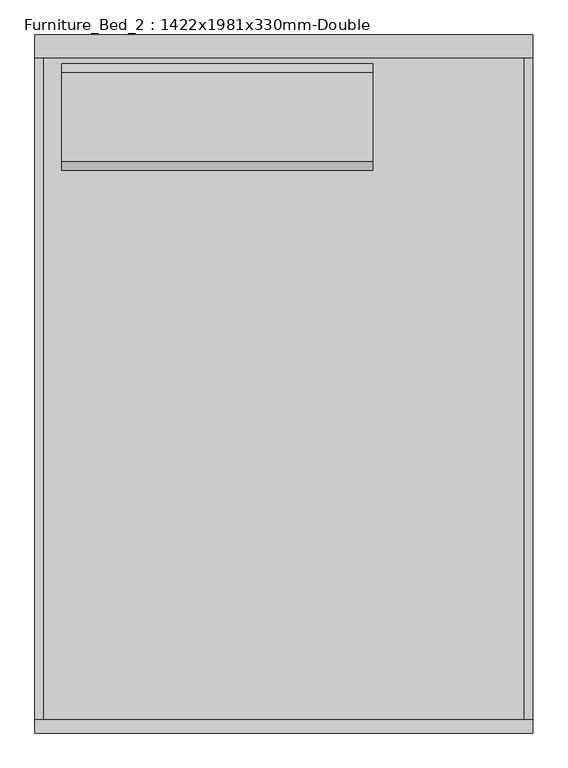
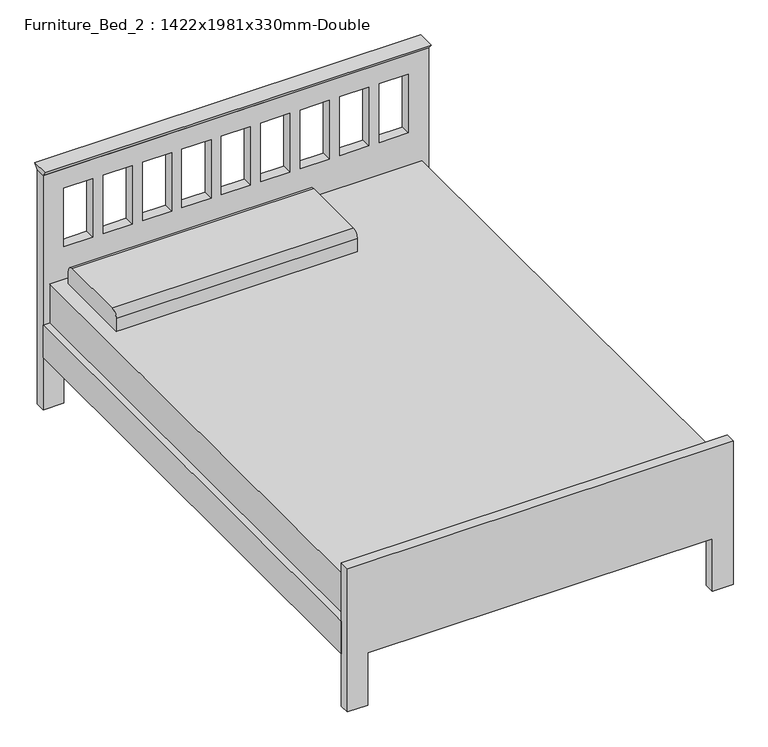
"""IFC4 building model written with IfcOpenShell, lengths in millimetres: furniture geometry, Furniture_Bed_2 : 1422x1981x330mm-Double."""

import ifcopenshell
import ifcopenshell.guid

model = None  # the IFC model being written
_history = None  # IfcOwnerHistory: only IFC2X3 demands one
_inside = {}  # id of a spatial element -> (the spatial element, [elements in it])
_under = {}  # id of a project, library or spatial element -> (it, [spatial elements below it])
_declared = {}  # id of a project -> (the project, [libraries it declares])
_typed = {}  # id of a type object -> (the type object, [elements of that type])
_made_of = {}  # id of a material, layer set ... -> (it, [elements and type objects made of it])


def new_model(schema):
    """Start an empty IFC model of exactly this schema.

    Asked for "IFC4X3", IfcOpenShell would pick the latest addendum, in which some entities
    have other attributes; the version numbers below select the first issue.
    IFC2X3 requires an IfcOwnerHistory on every rooted entity: one is made here for all.
    """
    global model, _history
    if schema == "IFC4X3":
        model = ifcopenshell.file(schema_version=(4, 3, 0, 0))
    else:
        model = ifcopenshell.file(schema=schema)
    _inside.clear()
    _under.clear()
    _declared.clear()
    _typed.clear()
    _made_of.clear()
    _history = None
    if model.schema == "IFC2X3":
        org = make("IfcOrganization", Name="unknown")
        user = make(
            "IfcPersonAndOrganization",
            ThePerson=make("IfcPerson", FamilyName="unknown"),
            TheOrganization=org,
        )
        app = make(
            "IfcApplication",
            ApplicationDeveloper=org,
            Version="unknown",
            ApplicationFullName="unknown",
            ApplicationIdentifier="unknown",
        )
        _history = make(
            "IfcOwnerHistory",
            OwningUser=user,
            OwningApplication=app,
            ChangeAction="ADDED",
            CreationDate=0,
        )
    return model


def make(cls, **values):
    """One entity of the class cls with the attributes given. An attribute that is None is left unset."""
    return model.create_entity(
        cls, **{name: value for name, value in values.items() if value is not None}
    )


def rooted(cls, **values):
    """An entity with a GlobalId (a new one), such as an element, a storey or a relation."""
    return make(cls, GlobalId=ifcopenshell.guid.new(), OwnerHistory=_history, **values)


def si_unit(unit_type, name, prefix=None):
    """IfcSIUnit, for example si_unit("LENGTHUNIT", "METRE", prefix="MILLI")."""
    return make("IfcSIUnit", UnitType=unit_type, Prefix=prefix, Name=name)


def assignment(units):
    """IfcUnitAssignment: the units of a project."""
    return None if units is None else make("IfcUnitAssignment", Units=units)


def point(xyz):
    """IfcCartesianPoint."""
    return None if xyz is None else make("IfcCartesianPoint", Coordinates=xyz)


def direction(xyz):
    """IfcDirection."""
    return None if xyz is None else make("IfcDirection", DirectionRatios=xyz)


def frame(location, z_axis=None, x_axis=None):
    """IfcAxis2Placement3D, a coordinate frame: its origin and axes. An axis left out is left unset."""
    return make(
        "IfcAxis2Placement3D",
        Location=point(location),
        Axis=direction(z_axis),
        RefDirection=direction(x_axis),
    )


def frame_2d(location, x_axis=None):
    """IfcAxis2Placement2D, a coordinate frame in the plane: its origin and x axis."""
    return make(
        "IfcAxis2Placement2D", Location=point(location), RefDirection=direction(x_axis)
    )


def origin():
    """The frame at (0, 0, 0) with its axes left unset."""
    return frame((0.0, 0.0, 0.0))


def place(relative_to, where):
    """IfcLocalPlacement: puts the frame where relative to a parent placement (None: the world)."""
    return make(
        "IfcLocalPlacement", PlacementRelTo=relative_to, RelativePlacement=where
    )


def context(
    kind, dimensions, precision=None, world=None, true_north=None, identifier=None
):
    """IfcGeometricRepresentationContext, for example the 3D "Model" context."""
    return make(
        "IfcGeometricRepresentationContext",
        ContextIdentifier=identifier,
        ContextType=kind,
        CoordinateSpaceDimension=dimensions,
        Precision=precision,
        WorldCoordinateSystem=world,
        TrueNorth=true_north,
    )


def project(units=None, contexts=None):
    """IfcProject with its units and contexts."""
    return rooted(
        "IfcProject",
        Name="project",
        RepresentationContexts=contexts,
        UnitsInContext=assignment(units),
    )


def spatial(cls, under=None, at=None, **own):
    """A site, building, storey or space (cls), placed at a placement, below another one or the project."""
    s = rooted(cls, ObjectPlacement=at, **own)
    if under is not None:
        _under.setdefault(under.id(), (under, []))[1].append(s)
    return s


def polyline(points):
    """IfcPolyline through the points."""
    return make("IfcPolyline", Points=[point(p) for p in points])


def circle_curve(where, radius):
    """IfcCircle in the frame where."""
    return make("IfcCircle", Position=where, Radius=radius)


def trimmed(basis, trim1, trim2, sense, master):
    """IfcTrimmedCurve: the piece of a basis curve between two trims."""
    return make(
        "IfcTrimmedCurve",
        BasisCurve=basis,
        Trim1=trim1,
        Trim2=trim2,
        SenseAgreement=sense,
        MasterRepresentation=master,
    )


def segment(curve, same_sense, transition):
    """IfcCompositeCurveSegment."""
    return make(
        "IfcCompositeCurveSegment",
        Transition=transition,
        SameSense=same_sense,
        ParentCurve=curve,
    )


def composite_curve(segments, self_intersect=None):
    """IfcCompositeCurve: segments joined end to end."""
    return make("IfcCompositeCurve", Segments=segments, SelfIntersect=self_intersect)


def outline(outer, holes=None, kind="AREA"):
    """IfcArbitraryClosedProfileDef: a profile drawn as a closed curve; with holes, ...WithVoids."""
    if holes is None:
        return make("IfcArbitraryClosedProfileDef", ProfileType=kind, OuterCurve=outer)
    return make(
        "IfcArbitraryProfileDefWithVoids",
        ProfileType=kind,
        OuterCurve=outer,
        InnerCurves=holes,
    )


def extrude(swept, where, along, depth):
    """IfcExtrudedAreaSolid: the profile swept, set in the frame where, extruded along a direction by depth."""
    return make(
        "IfcExtrudedAreaSolid",
        SweptArea=swept,
        Position=where,
        ExtrudedDirection=direction(along),
        Depth=depth,
    )


def shape(context_of_items, identifier, shape_type, items):
    """IfcShapeRepresentation: the items that make up one representation, for example the "Body"."""
    return make(
        "IfcShapeRepresentation",
        ContextOfItems=context_of_items,
        RepresentationIdentifier=identifier,
        RepresentationType=shape_type,
        Items=items,
    )


def source(mapping_origin, context_of_items, identifier, shape_type, items):
    """IfcRepresentationMap: a shape defined once, which mapped items show again and again."""
    return make(
        "IfcRepresentationMap",
        MappingOrigin=mapping_origin,
        MappedRepresentation=shape(context_of_items, identifier, shape_type, items),
    )


def transform(
    local_origin,
    x_axis=None,
    y_axis=None,
    z_axis=None,
    scale=None,
    scale2=None,
    scale3=None,
    uniform=True,
):
    """IfcCartesianTransformationOperator3D, or its non-uniform kind. x_axis, y_axis, z_axis: its Axis1, 2, 3."""
    if uniform:
        return make(
            "IfcCartesianTransformationOperator3D",
            Axis1=direction(x_axis),
            Axis2=direction(y_axis),
            LocalOrigin=point(local_origin),
            Scale=scale,
            Axis3=direction(z_axis),
        )
    return make(
        "IfcCartesianTransformationOperator3DnonUniform",
        Axis1=direction(x_axis),
        Axis2=direction(y_axis),
        LocalOrigin=point(local_origin),
        Scale=scale,
        Axis3=direction(z_axis),
        Scale2=scale2,
        Scale3=scale3,
    )


def mapped(mapping_source, mapping_target):
    """IfcMappedItem: shows the shape of a source again, moved by a transform."""
    return make(
        "IfcMappedItem", MappingSource=mapping_source, MappingTarget=mapping_target
    )


def made_of(thing, what):
    """Note that an element or type object is made of a material, layer set ...; save() writes the relation."""
    if what is not None:
        _made_of.setdefault(what.id(), (what, []))[1].append(thing)
    return thing


def element(
    cls,
    number,
    at=None,
    inside=None,
    cuts=None,
    type_object=None,
    material=None,
    context=None,
    identifier="Body",
    shape_type=None,
    held_by="IfcProductDefinitionShape",
    body=None,
    shapes=None,
    **own,
):
    """One element of the class cls, such as IfcWall. Its Tag is "e" and its number.

    at: its placement. inside: the storey or other place that contains it. cuts: it is an
    opening in that element (IfcRelVoidsElement). A single representation is given by context,
    identifier, shape_type and body (its items); several are given by shapes. held_by: the class
    of the entity that holds the representations. save() writes the other relations.
    """
    e = rooted(cls, Tag="e%d" % number, ObjectPlacement=at, **own)
    if body is not None:
        shapes = [shape(context, identifier, shape_type, body)]
    if shapes is not None:
        e.Representation = make(held_by, Representations=shapes)
    if inside is not None:
        _inside.setdefault(inside.id(), (inside, []))[1].append(e)
    if cuts is not None:
        rooted(
            "IfcRelVoidsElement", RelatingBuildingElement=cuts, RelatedOpeningElement=e
        )
    if type_object is not None:
        _typed.setdefault(type_object.id(), (type_object, []))[1].append(e)
    return made_of(e, material)


def aggregate(whole, parts):
    """IfcRelAggregates: a whole, such as a stair, and the parts it consists of."""
    return rooted("IfcRelAggregates", RelatingObject=whole, RelatedObjects=parts)


def save(model, path):
    """Write the relations noted so far, then the file.

    IfcRelAggregates (storeys below a building ...), IfcRelContainedInSpatialStructure (elements
    in a storey), IfcRelDefinesByType, IfcRelAssociatesMaterial and IfcRelDeclares: one each for
    every whole, place, type object, material and project.
    """
    for whole, parts in _under.values():
        aggregate(whole, parts)
    for where, things in _inside.values():
        rooted(
            "IfcRelContainedInSpatialStructure",
            RelatedElements=things,
            RelatingStructure=where,
        )
    for kind, things in _typed.values():
        rooted("IfcRelDefinesByType", RelatedObjects=things, RelatingType=kind)
    for what, things in _made_of.values():
        rooted("IfcRelAssociatesMaterial", RelatedObjects=things, RelatingMaterial=what)
    for by, libraries in _declared.values():
        rooted("IfcRelDeclares", RelatingContext=by, RelatedDefinitions=libraries)
    model.write(path)


def furniture_bed_2_1422x1981x330mm_double_4b4b7670(model_context):
    return source(origin(), model_context, "Body", "SweptSolid", [
        extrude(outline(polyline([(-38.1, 914.4), (-51.9545455, 933.45), (13.8545455, 933.45), (0.0, 914.4), (-38.1, 914.4)])), frame((-730.0365546, 0.0, 0.0), z_axis=(1.0, 0.0, 0.0), x_axis=(0.0, 1.0, 0.0)), (0.0, 0.0, 1.0), 1422.4533613),
        extrude(outline(composite_curve([segment(polyline([(-373.2486637, 482.6), (-373.2486637, 533.4)]), True, "CONTINUOUS"), segment(trimmed(circle_curve(frame_2d((-347.8486637, 533.4)), 25.4), [point((-373.2486637, 533.4))], [point((-347.8486637, 558.8))], False, "CARTESIAN"), True, "CONTINUOUS"), segment(polyline([(-347.8486637, 558.8), (-93.8486637, 558.8)]), True, "CONTINUOUS"), segment(trimmed(circle_curve(frame_2d((-93.8486637, 533.4)), 25.4), [point((-93.8486637, 558.8))], [point((-68.4486637, 533.4))], False, "CARTESIAN"), True, "CONTINUOUS"), segment(polyline([(-68.4486637, 533.4), (-68.4486637, 482.6), (-373.2486637, 482.6)]), True, "CONTINUOUS")], self_intersect=False)), frame((-654.05, 0.0, 0.0), z_axis=(1.0, 0.0, 0.0), x_axis=(0.0, 1.0, 0.0)), (0.0, 0.0, 1.0), 889.0),
        extrude(outline(polyline([(666.75, -38.1), (666.75, -1943.1), (-704.85, -1943.1), (-704.85, -38.1), (666.75, -38.1)])), frame((0.0, 0.0, 228.6), z_axis=(0.0, 0.0, 1.0), x_axis=(1.0, 0.0, 0.0)), (0.0, 0.0, 1.0), 254.0),
        extrude(outline(polyline([(666.75, -1943.1), (666.75, -38.1), (692.15, -38.1), (692.15, -1943.1), (666.75, -1943.1)])), frame((0.0, 0.0, 203.0994861), z_axis=(0.0, 0.0, 1.0), x_axis=(1.0, 0.0, 0.0)), (0.0, 0.0, 1.0), 127.0),
        extrude(outline(polyline([(-730.25, -1943.1), (-730.25, -38.1), (-704.85, -38.1), (-704.85, -1943.1), (-730.25, -1943.1)])), frame((0.0, 0.0, 203.5755296), z_axis=(0.0, 0.0, 1.0), x_axis=(1.0, 0.0, 0.0)), (0.0, 0.0, 1.0), 127.0),
        extrude(outline(polyline([(0.0, -654.05), (203.2, -654.05), (203.2, 615.95), (0.0, 615.95), (0.0, 692.15), (558.8, 692.15), (558.8, -730.25), (0.0, -730.25), (0.0, -654.05)])), frame((0.0, -1981.2, 0.0), z_axis=(0.0, 1.0, 0.0), x_axis=(0.0, 0.0, 1.0)), (0.0, 0.0, 1.0), 38.1),
        extrude(outline(polyline([(914.4, 692.4168067), (914.4, -730.0365546), (0.0, -730.0365546), (0.0, -654.05), (203.2, -654.05), (203.2, 234.95), (0.0, 234.95), (0.0, 692.4168067), (914.4, 692.4168067)]), holes=[polyline([(838.2, -546.8055556), (609.6, -546.8055556), (609.6, -654.05), (838.2, -654.05), (838.2, -546.8055556)]), polyline([(838.2, -401.4611111), (609.6, -401.4611111), (609.6, -508.7055556), (838.2, -508.7055556), (838.2, -401.4611111)]), polyline([(838.2, -256.1166667), (609.6, -256.1166667), (609.6, -363.3611111), (838.2, -363.3611111), (838.2, -256.1166667)]), polyline([(838.2, -110.7722222), (609.6, -110.7722222), (609.6, -218.0166667), (838.2, -218.0166667), (838.2, -110.7722222)]), polyline([(838.2, 179.9166667), (609.6, 179.9166667), (609.6, 72.6722222), (838.2, 72.6722222), (838.2, 179.9166667)]), polyline([(838.2, 325.2611111), (609.6, 325.2611111), (609.6, 218.0166667), (838.2, 218.0166667), (838.2, 325.2611111)]), polyline([(838.2, 470.6055556), (609.6, 470.6055556), (609.6, 363.3611111), (838.2, 363.3611111), (838.2, 470.6055556)]), polyline([(838.2, 615.95), (609.6, 615.95), (609.6, 508.7055556), (838.2, 508.7055556), (838.2, 615.95)]), polyline([(838.2, 34.5722222), (609.6, 34.5722222), (609.6, -72.6722222), (838.2, -72.6722222), (838.2, 34.5722222)])]), frame((0.0, -38.1, 0.0), z_axis=(0.0, 1.0, 0.0), x_axis=(0.0, 0.0, 1.0)), (0.0, 0.0, 1.0), 38.1),
    ])


if __name__ == "__main__":
    model = new_model("IFC4")
    model_context = context("Model", 3, world=origin())
    ifc_project = project(units=[si_unit("LENGTHUNIT", "METRE", prefix="MILLI")], contexts=[model_context])
    site = spatial("IfcSite", under=ifc_project)
    building = spatial("IfcBuilding", under=site)
    placement = place(None, origin())
    furniture_bed_2_1422x1981x330mm_double_shape = furniture_bed_2_1422x1981x330mm_double_4b4b7670(model_context)
    element("IfcFurniture", 1, ObjectType="Furniture_Bed_2 : 1422x1981x330mm-Double", at=placement, inside=building, context=model_context, shape_type="MappedRepresentation", body=[
        mapped(furniture_bed_2_1422x1981x330mm_double_shape, transform((0.0, 0.0, 0.0), x_axis=(1.0, 0.0, 0.0), y_axis=(0.0, 1.0, 0.0), z_axis=(0.0, 0.0, 1.0))),
    ])
    save(model, "model.ifc")

# Revit data of these elements
# Type "Furniture_Bed_2 : 1422x1981x330mm-Double"
#   Keynote = "N"
#   Length = 1981.2 mm
#   Width = 1422.4 mm
#   Material Frame = Wood - Birch
#   Material Mattress = Textile - White
# Element 1 (IfcFurniture, "Furniture_Bed_2 : 1422x1981x330mm-Double")
#   Materials on its faces: "Wood - Birch", "Textile - White"
# Materials
#   "Wood - Birch": class "Wood", colour RGB 224 178 126, transparency 0
#   "Textile - White": class "Fabric", colour RGB 247 247 239, transparency 0
